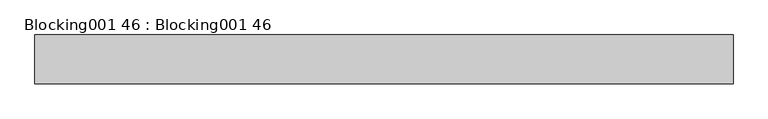
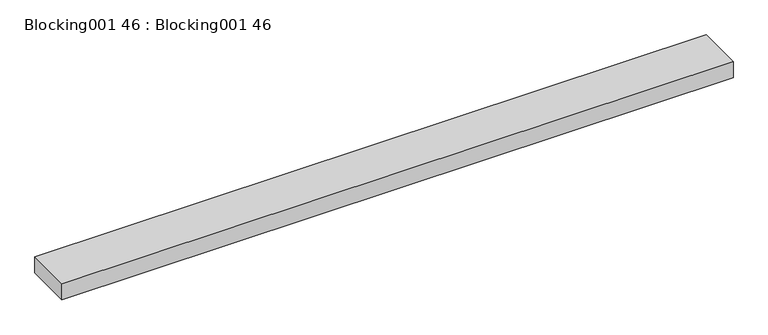
"""IFC4 building model written with IfcOpenShell, lengths in millimetres: proxy geometry, Blocking001 46 : Blocking001 46."""

from ifc_helpers import new_model, si_unit, frame, origin, place, context, project, spatial, polyline, outline, extrude, source, transform, mapped, element, save


def blocking001_46_blocking001_46_bc02a0c2(model_context):
    return source(origin(), model_context, "Body", "SweptSolid", [
        extrude(outline(polyline([(3694.2883192, 10278.0250834), (3694.2883192, 10417.7250834), (5694.2883192, 10417.7250834), (5694.2883192, 10278.0250834), (3694.2883192, 10278.0250834)])), frame((0.0, 0.0, 40722.296), z_axis=(0.0, 0.0, 1.0), x_axis=(1.0, 0.0, 0.0)), (0.0, 0.0, 1.0), 50.8),
    ])


if __name__ == "__main__":
    model = new_model("IFC4")
    model_context = context("Model", 3, world=origin())
    ifc_project = project(units=[si_unit("LENGTHUNIT", "METRE", prefix="MILLI")], contexts=[model_context])
    site = spatial("IfcSite", under=ifc_project)
    building = spatial("IfcBuilding", under=site)
    placement = place(None, origin())
    blocking001_46_blocking001_46_shape = blocking001_46_blocking001_46_bc02a0c2(model_context)
    element("IfcBuildingElementProxy", 1, Name="Blocking001 46 : Blocking001 46", ObjectType="Blocking001 46 : Blocking001 46", at=placement, inside=building, context=model_context, shape_type="MappedRepresentation", body=[
        mapped(blocking001_46_blocking001_46_shape, transform((0.0, 0.0, 0.0), x_axis=(1.0, 0.0, 0.0), y_axis=(0.0, 1.0, 0.0), z_axis=(0.0, 0.0, 1.0))),
    ])
    save(model, "model.ifc")

# Revit data of these elements
# Type "Blocking001 46 : Blocking001 46"
#   NameOverride = "Blocking001"
# Element 1 (IfcBuildingElementProxy, "Blocking001 46 : Blocking001 46")
#   Materials on its faces: "WOOD BLOCKING AS REQUIRED"
# Materials
#   "WOOD BLOCKING AS REQUIRED": class "Unassigned", colour RGB 166 124 85, transparency 0, Cost = 0
